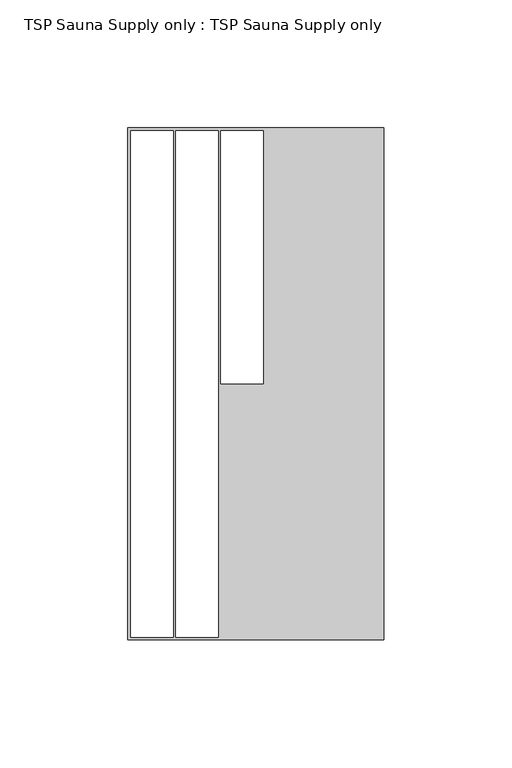
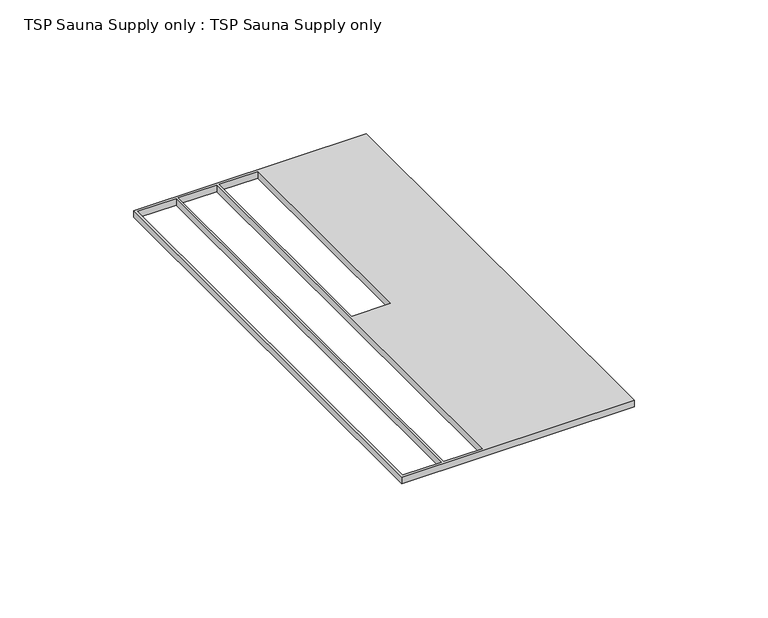
"""IFC4 building model written with IfcOpenShell, lengths in millimetres: proxy geometry, TSP Sauna Supply only : TSP Sauna Supply only."""

from ifc_helpers import new_model, si_unit, origin, origin_with_axes, place, context, project, spatial, polyline, outline, extrude, source, transform, mapped, element, save


def tsp_sauna_supply_only_tsp_sauna_supply_only_7ae9fcc8(model_context):
    return source(origin(), model_context, "Body", "SweptSolid", [
        extrude(outline(polyline([(-100.0, 100.0), (0.0, 100.0), (0.0, -100.0), (-100.0, -100.0), (-100.0, 100.0)]), holes=[polyline([(-99.0, -99.0), (-82.4142136, -99.0), (-82.4142136, 99.0), (-99.0, 99.0), (-99.0, -99.0)]), polyline([(-81.4142136, -99.0), (-64.8284271, -99.0), (-64.8284271, 99.0), (-81.4142136, 99.0), (-81.4142136, -99.0)]), polyline([(-63.8284271, 0.0), (-47.2426407, 0.0), (-47.2426407, 99.0), (-63.8284271, 99.0), (-63.8284271, 0.0)])]), origin_with_axes(), (0.0, 0.0, 1.0), 3.0),
    ])


if __name__ == "__main__":
    model = new_model("IFC4")
    model_context = context("Model", 3, world=origin())
    ifc_project = project(units=[si_unit("LENGTHUNIT", "METRE", prefix="MILLI")], contexts=[model_context])
    site = spatial("IfcSite", under=ifc_project)
    building = spatial("IfcBuilding", under=site)
    placement = place(None, origin())
    tsp_sauna_supply_only_tsp_sauna_supply_only_shape = tsp_sauna_supply_only_tsp_sauna_supply_only_7ae9fcc8(model_context)
    element("IfcBuildingElementProxy", 1, Name="TSP Sauna Supply only : TSP Sauna Supply only", ObjectType="TSP Sauna Supply only : TSP Sauna Supply only", at=placement, inside=building, context=model_context, shape_type="MappedRepresentation", body=[
        mapped(tsp_sauna_supply_only_tsp_sauna_supply_only_shape, transform((0.0, 0.0, 0.0), x_axis=(1.0, 0.0, 0.0), y_axis=(0.0, 1.0, 0.0), z_axis=(0.0, 0.0, 1.0))),
    ])
    save(model, "model.ifc")

# Revit data of these elements
# Type "TSP Sauna Supply only : TSP Sauna Supply only"
#   Model = "TSP_ELECSAUS"
#   Default Elevation = 0
# Element 1 (IfcBuildingElementProxy, "TSP Sauna Supply only : TSP Sauna Supply only")
#   Materials on its faces: "Plastic, Opaque Black"
# Materials
#   "Plastic, Opaque Black": class "Plastic", colour RGB 0 0 0, transparency 0.7, Description = "Plastic, generic, opaque black", Cost = 0
